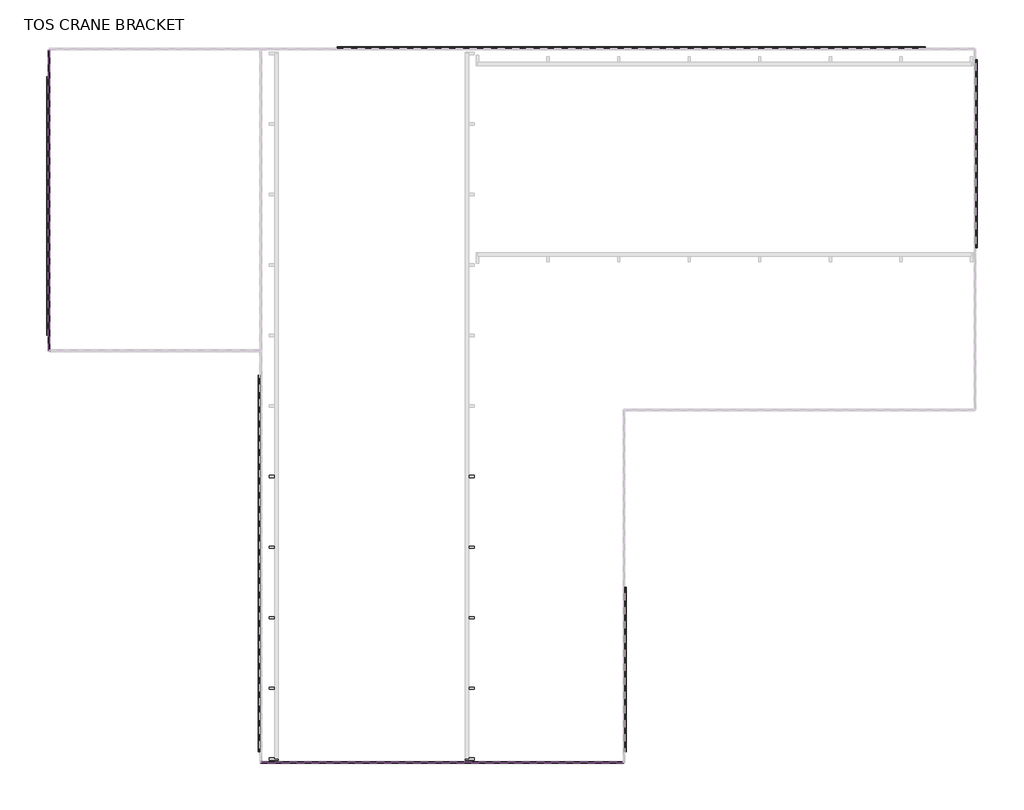
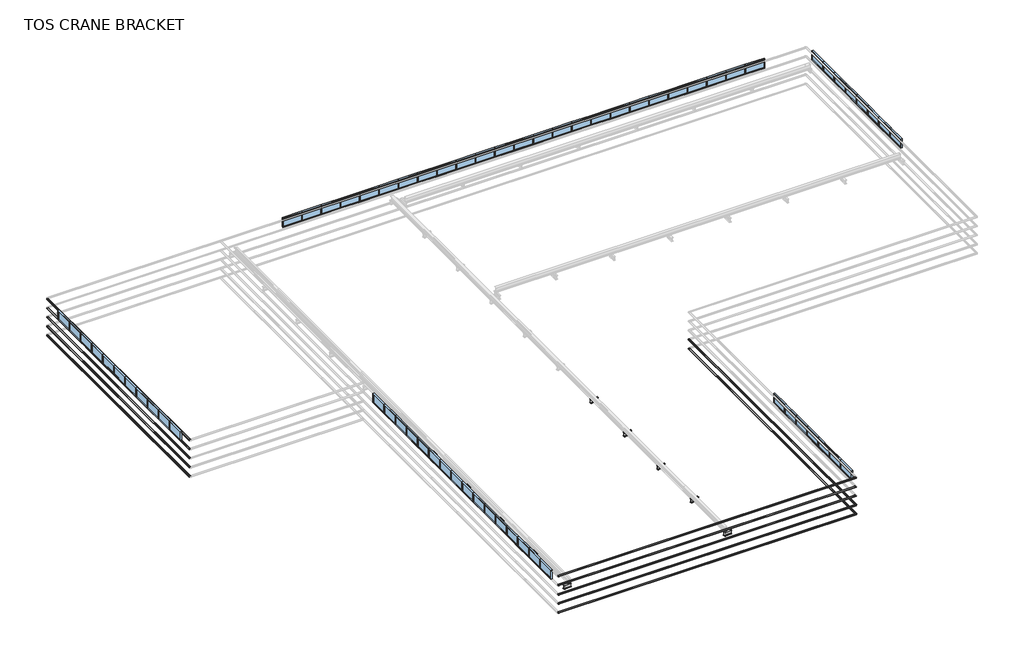
# One storey, part 1 of 3: 67 windows, 22 beams.
# Revit data of these elements (continued)
# Grids (mm) (continued)
#   "J": line (-13391.6, -54000) -> (49655.237, -54000)
#   "K": line (-13391.6, -60000) -> (49655.237, -60000)
#   "D": line (-13391.6, -18000) -> (80462.842, -18000)
#   "L": line (57000, -16617.432) -> (57000, -33057.804)
#   "M": line (15000, -45000) -> (49655.237, -45000)
#   "N": line (3000, 1013.268) -> (3000, -707.321)
#   "O": line (9000, 1013.268) -> (9000, -707.321)
#   "P": line (15000, 1013.268) -> (15000, -707.321)
#   "Q": line (21000, 1013.268) -> (21000, -707.321)
#   "R": line (27000, 1013.268) -> (27000, -707.321)
#   "S": line (33000, 1013.268) -> (33000, -707.321)
#   "T": line (39000, 1013.268) -> (39000, -707.321)
#   "U": line (45000, 1013.268) -> (45000, -707.321)
#   "V": line (51000, 1013.268) -> (51000, -707.321)
#   "W": line (57000, 1013.268) -> (57000, -707.321)
#   "X": line (63000, 1013.268) -> (63000, -707.321)
#   "Y": line (69000, 1013.268) -> (69000, -707.321)
#   "Z": line (75000, 1013.268) -> (75000, -707.321)
#   "AA": line (-1254.065, -3000) -> (600, -3000)
#   "BB": line (-1254.065, -9000) -> (600, -9000)
#   "CC": line (-1254.065, -15000) -> (600, -15000)
#   "DD": line (-1254.065, -21500) -> (600, -21500)
#   "EE": line (16745.935, -27000) -> (18600, -27000)
#   "FF": line (16745.935, -33000) -> (18600, -33000)
#   "GG": line (16745.935, -39000) -> (18600, -39000)
#   "HH": line (16745.935, -45000) -> (18600, -45000)
#   "II": line (16745.935, -51000) -> (18600, -51000)
#   "JJ": line (16745.935, -57000) -> (18600, -57000)
# Type "Steel Framing_H_KS : H_SB_AR_S02_H-400x200x8x13_SCB1"
#   Type Comments = "MAIN"
#   Type Mark = "SCB1"
#   H_SectionID = "H-400x200x8x13"
#   H_Ratio for Additional Steel Plate = 0.2
#   Width = 20.0 cm
#   Web Thickness = 0.8 cm
#   Web Fillet = 1.6 cm
#   Warping Constant = 649000.0 cm⁶
#   Torsional Moment of Inertia = 35.8981 cm⁴
#   Section Area = 84.12 cm²
#   Plastic Modulus weak axis = 268.0 cm³
#   Plastic Modulus strong axis = 1330.0 cm³
#   Perimeter = 1.56 m²/m
#   Nominal Weight = 66.00 kgf/m
#   Moment of Inertia weak axis = 1740.00 cm⁴
#   Moment of Inertia strong axis = 23700.00 cm⁴
#   Height = 40.0 cm
#   Flange Thickness = 1.3 cm
#   Elastic Modulus weak axis = 174.0 cm³
#   Elastic Modulus strong axis = 1190.0 cm³
#   Centroid Vertical = 20.0 cm
#   Centroid Horizontal = 10.0 cm
#   Bolt Spacing = 8.89 cm
#   Length [instance default] = 1500 mm
#   Structural Material [instance default] = Steel, 45-345
#   Section Name Key = ""
#   Assembly Code = ""
# Type "Steel Framing_LC : H_SB_AR_S00_LC-150x75x25x3.2"
#   Type Comments = "SECONDARY"
#   Type Mark = "GIRTH"
#   H_SectionID = "LC-150x75x25x3.2"
#   r = 4.8 mm
#   d = 25 mm
#   R = 8 mm
#   Perimeter = 0.70 m²/m
#   Nominal Weight = 10.30 kgf/m
#   Length [instance default] = 1000 mm
#   b = 75 mm
#   h = 150 mm
#   tw = 3.2 mm
#   x = 18.6 mm
#   A = 1.00 m²
#   Structural Material [instance default] = Steel, 45-345
#   Assembly Code = ""
# Type "Fixed Window : H_WD_AR_B11_Fix_Steel Window_SG_W2000xH1000"
#   Description = "PVC Frame + 2 x T=6mm + T12mm Air Space"
#   Type Mark = "AW"
#   Analytic Construction = "<None>"
#   창 두께 = 150 mm
#   Height = 1000 mm
#   절반 창 두께 = 75 mm
#   기본 씰 높이 = 800 mm
#   Width = 2000 mm
#   Define Thermal Properties by = 1
#   창 패널 = none
#   창 프레임 = none
#   Wall Closure = (empty or 0)
# Elements 1, 2, 3, 4, 5, 6, 7, 8, 9, 10 (IfcBeam, "Steel Framing_H_KS : H_SB_AR_S02_H-400x200x8x13_SCB1")
#   Structural Material = Steel, 45-345
#   Phase Created = New Construction
#   Materials on its faces: "Steel, 45-345"
# Elements 11, 12, 13, 14, 15, 16, 17, 18, 19, 20, 21, 22 (IfcBeam, "Steel Framing_LC : H_SB_AR_S00_LC-150x75x25x3.2")
#   Structural Material = Steel, 45-345
#   Phase Created = New Construction
#   Materials on its faces: "Steel, 45-345"
# Element 23 (IfcWindow, "Fixed Window : H_WD_AR_B11_Fix_Steel Window_SG_W2000xH1000")
#   Mark = "02"
#   Phase Created = New Construction
# Element 24 (IfcWindow, "Fixed Window : H_WD_AR_B11_Fix_Steel Window_SG_W2000xH1000")
#   Mark = "03"
#   Phase Created = New Construction
# Element 25 (IfcWindow, "Fixed Window : H_WD_AR_B11_Fix_Steel Window_SG_W2000xH1000")
#   Mark = "04"
#   Phase Created = New Construction
# Element 26 (IfcWindow, "Fixed Window : H_WD_AR_B11_Fix_Steel Window_SG_W2000xH1000")
#   Mark = "05"
#   Phase Created = New Construction
# Element 27 (IfcWindow, "Fixed Window : H_WD_AR_B11_Fix_Steel Window_SG_W2000xH1000")
#   Mark = "06"
#   Phase Created = New Construction
# Element 28 (IfcWindow, "Fixed Window : H_WD_AR_B11_Fix_Steel Window_SG_W2000xH1000")
#   Mark = "07"
#   Phase Created = New Construction
# Element 29 (IfcWindow, "Fixed Window : H_WD_AR_B11_Fix_Steel Window_SG_W2000xH1000")
#   Mark = "08"
#   Phase Created = New Construction
# Element 30 (IfcWindow, "Fixed Window : H_WD_AR_B11_Fix_Steel Window_SG_W2000xH1000")
#   Mark = "09"
#   Phase Created = New Construction
# Element 31 (IfcWindow, "Fixed Window : H_WD_AR_B11_Fix_Steel Window_SG_W2000xH1000")
#   Mark = "10"
#   Phase Created = New Construction
# Element 32 (IfcWindow, "Fixed Window : H_WD_AR_B11_Fix_Steel Window_SG_W2000xH1000")
#   Mark = "11"
#   Phase Created = New Construction
# Element 33 (IfcWindow, "Fixed Window : H_WD_AR_B11_Fix_Steel Window_SG_W2000xH1000")
#   Mark = "12"
#   Phase Created = New Construction
# Element 34 (IfcWindow, "Fixed Window : H_WD_AR_B11_Fix_Steel Window_SG_W2000xH1000")
#   Mark = "13"
#   Phase Created = New Construction
# Element 35 (IfcWindow, "Fixed Window : H_WD_AR_B11_Fix_Steel Window_SG_W2000xH1000")
#   Mark = "14"
#   Phase Created = New Construction
# Element 36 (IfcWindow, "Fixed Window : H_WD_AR_B11_Fix_Steel Window_SG_W2000xH1000")
#   Mark = "15"
#   Phase Created = New Construction
# Element 37 (IfcWindow, "Fixed Window : H_WD_AR_B11_Fix_Steel Window_SG_W2000xH1000")
#   Mark = "16"
#   Phase Created = New Construction
# Element 38 (IfcWindow, "Fixed Window : H_WD_AR_B11_Fix_Steel Window_SG_W2000xH1000")
#   Mark = "17"
#   Phase Created = New Construction
# Element 39 (IfcWindow, "Fixed Window : H_WD_AR_B11_Fix_Steel Window_SG_W2000xH1000")
#   Mark = "18"
#   Phase Created = New Construction
# Element 40 (IfcWindow, "Fixed Window : H_WD_AR_B11_Fix_Steel Window_SG_W2000xH1000")
#   Mark = "19"
#   Phase Created = New Construction
# Element 41 (IfcWindow, "Fixed Window : H_WD_AR_B11_Fix_Steel Window_SG_W2000xH1000")
#   Mark = "20"
#   Phase Created = New Construction
# Element 42 (IfcWindow, "Fixed Window : H_WD_AR_B11_Fix_Steel Window_SG_W2000xH1000")
#   Mark = "21"
#   Phase Created = New Construction
# Element 43 (IfcWindow, "Fixed Window : H_WD_AR_B11_Fix_Steel Window_SG_W2000xH1000")
#   Mark = "22"
#   Phase Created = New Construction
# Element 44 (IfcWindow, "Fixed Window : H_WD_AR_B11_Fix_Steel Window_SG_W2000xH1000")
#   Mark = "23"
#   Phase Created = New Construction
# Element 45 (IfcWindow, "Fixed Window : H_WD_AR_B11_Fix_Steel Window_SG_W2000xH1000")
#   Mark = "24"
#   Phase Created = New Construction
# Element 46 (IfcWindow, "Fixed Window : H_WD_AR_B11_Fix_Steel Window_SG_W2000xH1000")
#   Mark = "25"
#   Phase Created = New Construction
# Element 47 (IfcWindow, "Fixed Window : H_WD_AR_B11_Fix_Steel Window_SG_W2000xH1000")
#   Mark = "26"
#   Phase Created = New Construction
# Element 48 (IfcWindow, "Fixed Window : H_WD_AR_B11_Fix_Steel Window_SG_W2000xH1000")
#   Mark = "27"
#   Phase Created = New Construction
# Element 49 (IfcWindow, "Fixed Window : H_WD_AR_B11_Fix_Steel Window_SG_W2000xH1000")
#   Mark = "28"
#   Phase Created = New Construction
# Element 50 (IfcWindow, "Fixed Window : H_WD_AR_B11_Fix_Steel Window_SG_W2000xH1000")
#   Mark = "29"
#   Phase Created = New Construction
# Element 51 (IfcWindow, "Fixed Window : H_WD_AR_B11_Fix_Steel Window_SG_W2000xH1000")
#   Mark = "30"
#   Phase Created = New Construction
# Element 52 (IfcWindow, "Fixed Window : H_WD_AR_B11_Fix_Steel Window_SG_W2000xH1000")
#   Mark = "31"
#   Phase Created = New Construction
# Element 53 (IfcWindow, "Fixed Window : H_WD_AR_B11_Fix_Steel Window_SG_W2000xH1000")
#   Mark = "32"
#   Phase Created = New Construction
# Element 54 (IfcWindow, "Fixed Window : H_WD_AR_B11_Fix_Steel Window_SG_W2000xH1000")
#   Mark = "33"
#   Phase Created = New Construction
# Element 55 (IfcWindow, "Fixed Window : H_WD_AR_B11_Fix_Steel Window_SG_W2000xH1000")
#   Mark = "34"
#   Phase Created = New Construction
# Element 56 (IfcWindow, "Fixed Window : H_WD_AR_B11_Fix_Steel Window_SG_W2000xH1000")
#   Mark = "35"
#   Phase Created = New Construction
# Element 57 (IfcWindow, "Fixed Window : H_WD_AR_B11_Fix_Steel Window_SG_W2000xH1000")
#   Mark = "36"
#   Phase Created = New Construction
# Element 58 (IfcWindow, "Fixed Window : H_WD_AR_B11_Fix_Steel Window_SG_W2000xH1000")
#   Mark = "37"
#   Phase Created = New Construction
# Element 59 (IfcWindow, "Fixed Window : H_WD_AR_B11_Fix_Steel Window_SG_W2000xH1000")
#   Mark = "38"
#   Phase Created = New Construction
# Element 60 (IfcWindow, "Fixed Window : H_WD_AR_B11_Fix_Steel Window_SG_W2000xH1000")
#   Mark = "39"
#   Phase Created = New Construction
# Element 61 (IfcWindow, "Fixed Window : H_WD_AR_B11_Fix_Steel Window_SG_W2000xH1000")
#   Mark = "40"
#   Phase Created = New Construction
# Element 62 (IfcWindow, "Fixed Window : H_WD_AR_B11_Fix_Steel Window_SG_W2000xH1000")
#   Mark = "41"
#   Phase Created = New Construction
# Element 63 (IfcWindow, "Fixed Window : H_WD_AR_B11_Fix_Steel Window_SG_W2000xH1000")
#   Mark = "42"
#   Phase Created = New Construction
# Element 64 (IfcWindow, "Fixed Window : H_WD_AR_B11_Fix_Steel Window_SG_W2000xH1000")
#   Mark = "43"
#   Phase Created = New Construction
# Element 65 (IfcWindow, "Fixed Window : H_WD_AR_B11_Fix_Steel Window_SG_W2000xH1000")
#   Mark = "44"
#   Phase Created = New Construction
# Element 66 (IfcWindow, "Fixed Window : H_WD_AR_B11_Fix_Steel Window_SG_W2000xH1000")
#   Mark = "45"
#   Phase Created = New Construction
# Element 67 (IfcWindow, "Fixed Window : H_WD_AR_B11_Fix_Steel Window_SG_W2000xH1000")
#   Mark = "46"
#   Phase Created = New Construction
# Element 68 (IfcWindow, "Fixed Window : H_WD_AR_B11_Fix_Steel Window_SG_W2000xH1000")
#   Mark = "47"
#   Phase Created = New Construction
# Element 69 (IfcWindow, "Fixed Window : H_WD_AR_B11_Fix_Steel Window_SG_W2000xH1000")
#   Mark = "48"
#   Phase Created = New Construction
# Element 70 (IfcWindow, "Fixed Window : H_WD_AR_B11_Fix_Steel Window_SG_W2000xH1000")
#   Mark = "49"
#   Phase Created = New Construction
# Element 71 (IfcWindow, "Fixed Window : H_WD_AR_B11_Fix_Steel Window_SG_W2000xH1000")
#   Mark = "50"
#   Phase Created = New Construction
# Element 72 (IfcWindow, "Fixed Window : H_WD_AR_B11_Fix_Steel Window_SG_W2000xH1000")
#   Mark = "51"
#   Phase Created = New Construction
# Element 73 (IfcWindow, "Fixed Window : H_WD_AR_B11_Fix_Steel Window_SG_W2000xH1000")
#   Mark = "52"
#   Phase Created = New Construction
# Element 74 (IfcWindow, "Fixed Window : H_WD_AR_B11_Fix_Steel Window_SG_W2000xH1000")
#   Mark = "53"
#   Phase Created = New Construction
# Element 75 (IfcWindow, "Fixed Window : H_WD_AR_B11_Fix_Steel Window_SG_W2000xH1000")
#   Mark = "54"
#   Phase Created = New Construction
# Element 76 (IfcWindow, "Fixed Window : H_WD_AR_B11_Fix_Steel Window_SG_W2000xH1000")
#   Mark = "55"
#   Phase Created = New Construction
# Element 77 (IfcWindow, "Fixed Window : H_WD_AR_B11_Fix_Steel Window_SG_W2000xH1000")
#   Mark = "56"
#   Phase Created = New Construction
# Element 78 (IfcWindow, "Fixed Window : H_WD_AR_B11_Fix_Steel Window_SG_W2000xH1000")
#   Mark = "57"
#   Phase Created = New Construction
# Element 79 (IfcWindow, "Fixed Window : H_WD_AR_B11_Fix_Steel Window_SG_W2000xH1000")
#   Mark = "58"
#   Phase Created = New Construction
# Element 80 (IfcWindow, "Fixed Window : H_WD_AR_B11_Fix_Steel Window_SG_W2000xH1000")
#   Mark = "59"
#   Phase Created = New Construction
# Element 81 (IfcWindow, "Fixed Window : H_WD_AR_B11_Fix_Steel Window_SG_W2000xH1000")
#   Mark = "60"
#   Phase Created = New Construction
# Element 82 (IfcWindow, "Fixed Window : H_WD_AR_B11_Fix_Steel Window_SG_W2000xH1000")
#   Mark = "61"
#   Phase Created = New Construction
# Element 83 (IfcWindow, "Fixed Window : H_WD_AR_B11_Fix_Steel Window_SG_W2000xH1000")
#   Mark = "62"
#   Phase Created = New Construction
# Element 84 (IfcWindow, "Fixed Window : H_WD_AR_B11_Fix_Steel Window_SG_W2000xH1000")
#   Mark = "63"
#   Phase Created = New Construction
# Element 85 (IfcWindow, "Fixed Window : H_WD_AR_B11_Fix_Steel Window_SG_W2000xH1000")
#   Mark = "64"
#   Phase Created = New Construction
# Element 86 (IfcWindow, "Fixed Window : H_WD_AR_B11_Fix_Steel Window_SG_W2000xH1000")
#   Mark = "65"
#   Phase Created = New Construction
# Element 87 (IfcWindow, "Fixed Window : H_WD_AR_B11_Fix_Steel Window_SG_W2000xH1000")
#   Mark = "66"
#   Phase Created = New Construction
# Element 88 (IfcWindow, "Fixed Window : H_WD_AR_B11_Fix_Steel Window_SG_W2000xH1000")
#   Mark = "67"
#   Phase Created = New Construction
# Element 89 (IfcWindow, "Fixed Window : H_WD_AR_B11_Fix_Steel Window_SG_W2000xH1000")
#   Mark = "68"
#   Phase Created = New Construction
# Materials
#   "Steel, 45-345": class "Metal", colour RGB 189 187 185, transparency 0, Description = "Steel 345 MPa", Cost = 0
